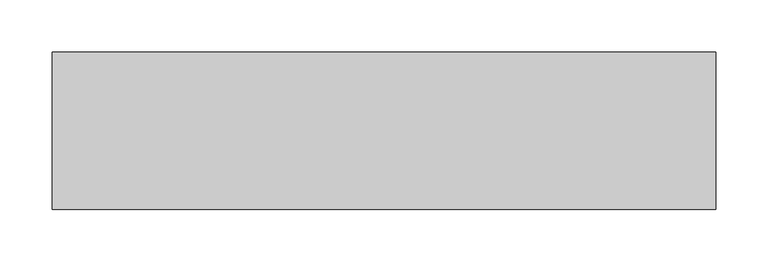
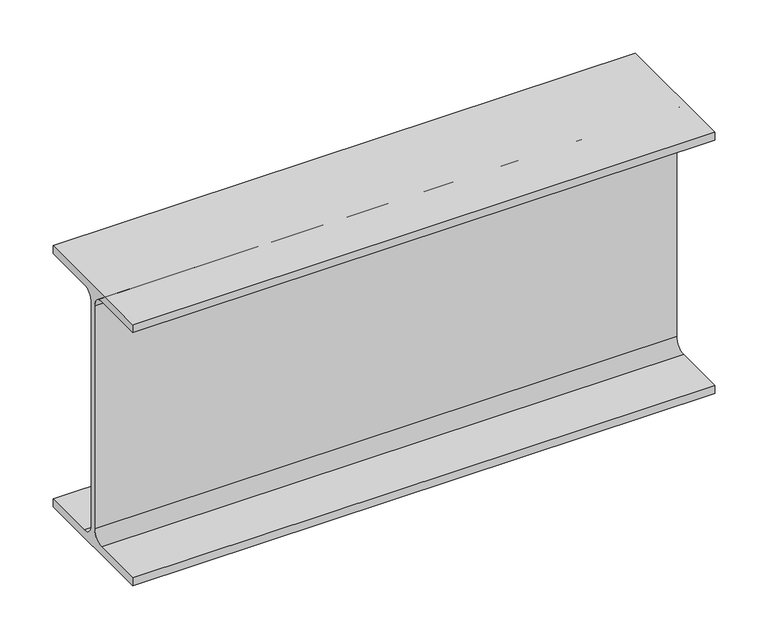
"""IFC4 building model written with IfcOpenShell, lengths in millimetres: beam geometry, 0912_Steel Framing_H-KSD3502 : H_SB_ASB_H-300x150x6.5x9."""

from ifc_helpers import new_model, si_unit, point, frame, frame_2d, origin, place, context, project, spatial, polyline, circle_curve, trimmed, segment, composite_curve, outline, extrude, source, transform, mapped, element, save


def beam_3d318208(model_context):
    return source(origin(), model_context, "Body", "SweptSolid", [
        extrude(outline(composite_curve([segment(polyline([(-75.0, -141.0), (-16.25, -141.0)]), True, "CONTINUOUS"), segment(trimmed(circle_curve(frame_2d((-16.25, -128.0)), 13.0), [point((-16.25, -141.0))], [point((-3.25, -128.0))], True, "CARTESIAN"), True, "CONTINUOUS"), segment(polyline([(-3.25, -128.0), (-3.25, 128.0)]), True, "CONTINUOUS"), segment(trimmed(circle_curve(frame_2d((-16.25, 128.0)), 13.0), [point((-3.25, 128.0))], [point((-16.25, 141.0))], True, "CARTESIAN"), True, "CONTINUOUS"), segment(polyline([(-16.25, 141.0), (-75.0, 141.0), (-75.0, 150.0), (75.0, 150.0), (75.0, 141.0), (16.25, 141.0)]), True, "CONTINUOUS"), segment(trimmed(circle_curve(frame_2d((16.25, 128.0)), 13.0), [point((16.25, 141.0))], [point((3.25, 128.0))], True, "CARTESIAN"), True, "CONTINUOUS"), segment(polyline([(3.25, 128.0), (3.25, -128.0)]), True, "CONTINUOUS"), segment(trimmed(circle_curve(frame_2d((16.25, -128.0)), 13.0), [point((3.25, -128.0))], [point((16.25, -141.0))], True, "CARTESIAN"), True, "CONTINUOUS"), segment(polyline([(16.25, -141.0), (75.0, -141.0), (75.0, -150.0), (-75.0, -150.0), (-75.0, -141.0)]), True, "CONTINUOUS")], self_intersect=False)), frame((-282.3, 0.0, 0.0), z_axis=(1.0, 0.0, 0.0), x_axis=(0.0, 1.0, 0.0)), (0.0, 0.0, 1.0), 632.1),
    ])


if __name__ == "__main__":
    model = new_model("IFC4")
    model_context = context("Model", 3, world=origin())
    ifc_project = project(units=[si_unit("LENGTHUNIT", "METRE", prefix="MILLI")], contexts=[model_context])
    site = spatial("IfcSite", under=ifc_project)
    building = spatial("IfcBuilding", under=site)
    placement = place(None, origin())
    beam_shape = beam_3d318208(model_context)
    element("IfcBeam", 1, ObjectType="0912_Steel Framing_H-KSD3502 : H_SB_ASB_H-300x150x6.5x9", at=placement, inside=building, context=model_context, shape_type="MappedRepresentation", body=[
        mapped(beam_shape, transform((0.0, 0.0, 0.0), x_axis=(1.0, 0.0, 0.0), y_axis=(0.0, 1.0, 0.0), z_axis=(0.0, 0.0, 1.0))),
    ])
    save(model, "model.ifc")

# Revit data of these elements
# Type "0912_Steel Framing_H-KSD3502 : H_SB_ASB_H-300x150x6.5x9"
#   H_WM Code_1 = "S01AA002-00001 | Main Steel Structure Fabrication Work | Shelter/Building | Medium Steel - Standard (90KG/M>Weight≥30KG/M) | Material: (   )"
#   H_WM Code_2 = "S03AA028-00001 | Main Steel Structure Erection Work | Shelter/Building | Medium Steel (90KG/M>Weight≥30KG/M) | Material: (   )"
#   H_WM Code_3 = "S01AA010-00001 | Main Steel Structure Fabrication Work | Shelter/Building | Steel Painting/Coating | for Non-Fireproofed Steel Surface, Surface Preparation, Primer, Second & Final Coat | Material: (   )"
#   H_Q'ty Cal Type Tag = "SB-Q2"
#   Width = 15.0 cm
#   Web Thickness = 0.65 cm
#   Web Fillet = 1.3 cm
#   Warping Constant = 107000.0 cm⁶
#   W = 0
#   Torsional Moment of Inertia = 9.9539 cm⁴
#   Section Area = 46.78 cm²
#   Plastic Modulus weak axis = 105.0 cm³
#   Plastic Modulus strong axis = 542.0 cm³
#   Perimeter = 1.17 m²/m
#   Nominal Weight = 36.70 kgf/m
#   Moment of Inertia weak axis = 508.00 cm⁴
#   Moment of Inertia strong axis = 7210.00 cm⁴
#   Height = 30.0 cm
#   Flange Thickness = 0.9 cm
#   Elastic Modulus weak axis = 67.7 cm³
#   Elastic Modulus strong axis = 481.0 cm³
#   Centroid Vertical = 15.0 cm
#   Centroid Horizontal = 7.5 cm
#   Ix = 72100000
#   Length [instance default] = 1.5240 m
#   Zx = 542000
#   b = 0.1500 m
#   h = 0.3000 m
#   r = 0.0130 m
#   s = 0.0065 m
#   t = 0.0090 m
#   A = 0.004678 m²
#   Structural Material [instance default] = Steel, 45-345
#   Assembly Code = ""
# Element 1 (IfcBeam, "0912_Steel Framing_H-KSD3502 : H_SB_ASB_H-300x150x6.5x9")
#   Structural Material = none
# Materials
#   "Steel, 45-345": class "Metal", colour RGB 189 187 185, transparency 0, Description = "Steel 345 MPa", Cost = 0
